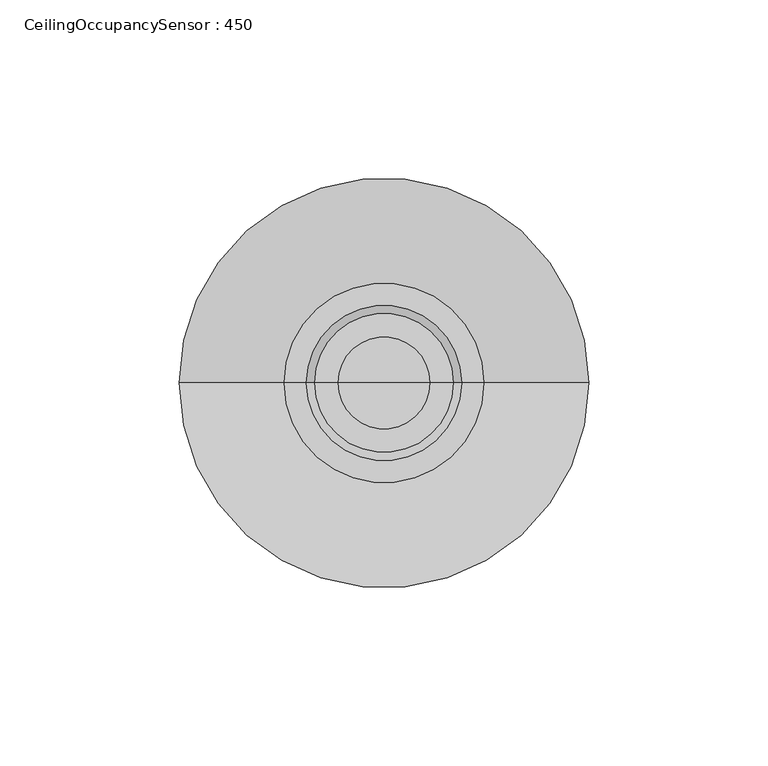
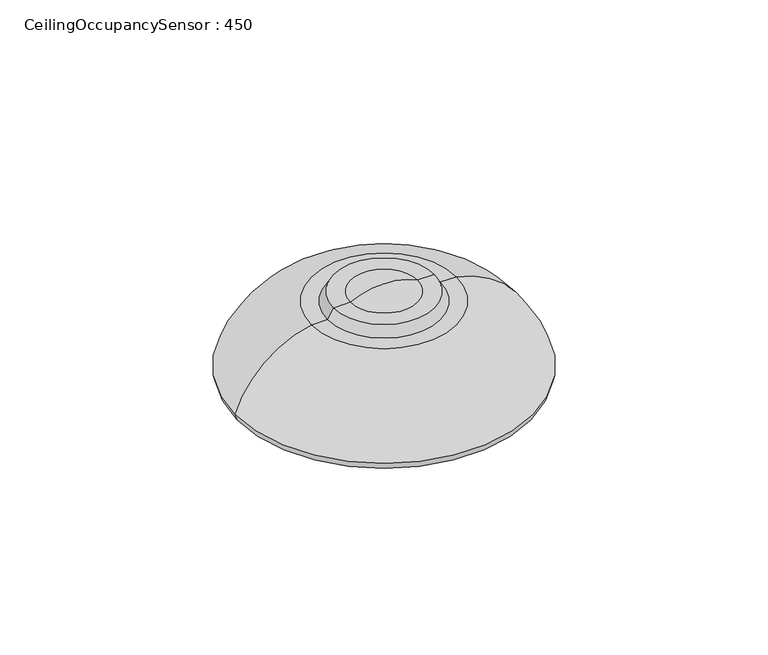
"""IFC4 building model written with IfcOpenShell, lengths in millimetres: switching device geometry, CeilingOccupancySensor : 450."""

from ifc_helpers import new_model, si_unit, point, frame, origin, origin_with_axes, place, context, project, spatial, polyline, circle_curve, ellipse_curve, trimmed, source, transform, mapped, element, save
from ifc_brep_helpers import plane_surface, revolved_surface, advanced_brep


def ceilingoccupancysensor_450_02cbfb90(model_context):
    return source(origin(), model_context, "Body", "AdvancedBrep", [
        advanced_brep(
        [(-12.7998992, 0.0, 32.54375), (12.7998992, 0.0, 32.54375), (0.0, 0.0, 35.5203125), (-19.3725919, 0.0, 32.54375), (19.3725919, 0.0, 32.54375), (-21.6519708, 0.0, 28.5957499), (21.6519708, 0.0, 28.5957499), (-27.834758, 0.0, 28.5957499), (27.834758, 0.0, 28.5957499), (-57.15, 0.0, 2.3911967), (57.15, 0.0, 2.3911967), (-56.5092808, 0.0, 0.0), (56.5092808, 0.0, 0.0), (0.0, 0.0, 0.0)],
        [
            (0, 1, circle_curve(frame((0.0, 0.0, 32.54375), z_axis=(0.0, 0.0, 1.0), x_axis=(1.0, 0.0, 0.0)), 12.7998992)),
            (1, 2, circle_curve(frame((0.750087, 0.0, 9.7363307), z_axis=(0.0, -1.0, 0.0), x_axis=(1.0, 0.0, 0.0)), 25.79489)),
            (2, 0, circle_curve(frame((-0.750087, 0.0, 9.7363307), z_axis=(0.0, -1.0, 0.0), x_axis=(-1.0, 0.0, 0.0)), 25.79489)),
            (1, 0, circle_curve(frame((0.0, 0.0, 32.54375), z_axis=(0.0, 0.0, 1.0), x_axis=(1.0, 0.0, 0.0)), 12.7998992)),
            (3, 4, circle_curve(frame((0.0, 0.0, 32.54375), z_axis=(0.0, 0.0, 1.0), x_axis=(1.0, 0.0, 0.0)), 19.3725919)),
            (4, 1),
            (0, 3),
            (4, 3, circle_curve(frame((0.0, 0.0, 32.54375), z_axis=(0.0, 0.0, 1.0), x_axis=(1.0, 0.0, 0.0)), 19.3725919)),
            (5, 6, circle_curve(frame((0.0, 0.0, 28.5957499), z_axis=(0.0, 0.0, 1.0), x_axis=(1.0, 0.0, 0.0)), 21.6519708)),
            (6, 4),
            (3, 5),
            (6, 5, circle_curve(frame((0.0, 0.0, 28.5957499), z_axis=(0.0, 0.0, 1.0), x_axis=(1.0, 0.0, 0.0)), 21.6519708)),
            (7, 8, circle_curve(frame((0.0, 0.0, 28.5957499), z_axis=(0.0, 0.0, 1.0), x_axis=(1.0, 0.0, 0.0)), 27.834758)),
            (8, 6),
            (5, 7),
            (8, 7, circle_curve(frame((0.0, 0.0, 28.5957499), z_axis=(0.0, 0.0, 1.0), x_axis=(1.0, 0.0, 0.0)), 27.834758)),
            (9, 10, circle_curve(frame((0.0, 0.0, 2.3911967), z_axis=(0.0, 0.0, 1.0), x_axis=(1.0, 0.0, 0.0)), 57.15)),
            (10, 8, circle_curve(frame((20.1846327, 0.0, -9.4623798), z_axis=(0.0, -1.0, 0.0), x_axis=(1.0, 0.0, 0.0)), 38.8193979)),
            (7, 9, circle_curve(frame((-20.1846327, 0.0, -9.4623798), z_axis=(0.0, -1.0, 0.0), x_axis=(-1.0, 0.0, 0.0)), 38.8193979)),
            (10, 9, circle_curve(frame((0.0, 0.0, 2.3911967), z_axis=(0.0, 0.0, 1.0), x_axis=(1.0, 0.0, 0.0)), 57.15)),
            (11, 12, circle_curve(origin_with_axes(), 56.5092808)),
            (12, 10),
            (9, 11),
            (12, 11, circle_curve(origin_with_axes(), 56.5092808)),
            (13, 12),
            (11, 13),
        ],
        [
            revolved_surface(trimmed(ellipse_curve(frame((0.750087, 0.0, 9.7363307), z_axis=(0.0, 1.0, 0.0), x_axis=(1.0, 0.0, 0.0)), 25.79489, 25.79489), [point((0.0, 0.0, 35.5203125))], [point((12.7998992, 0.0, 32.54375))], True, "CARTESIAN"), (0.0, 0.0, 38.1), (0.0, 0.0, -1.0)),
            plane_surface(frame((0.0, 0.0, 32.54375), z_axis=(0.0, 0.0, 1.0), x_axis=(1.0, 0.0, 0.0))),
            revolved_surface(polyline([(19.3725919, 0.0, 32.54375), (21.6519708, 0.0, 28.5957499)]), (0.0, 0.0, 38.1), (0.0, 0.0, -1.0)),
            plane_surface(frame((0.0, 0.0, 28.5957499), z_axis=(0.0, 0.0, 1.0), x_axis=(1.0, 0.0, 0.0))),
            revolved_surface(trimmed(ellipse_curve(frame((20.1846327, 0.0, -9.4623798), z_axis=(0.0, 1.0, 0.0), x_axis=(1.0, 0.0, 0.0)), 38.8193979, 38.8193979), [point((27.834758, 0.0, 28.5957499))], [point((57.15, 0.0, 2.3911967))], True, "CARTESIAN"), (0.0, 0.0, 38.1), (0.0, 0.0, -1.0)),
            revolved_surface(polyline([(57.15, 0.0, 2.3911967), (56.5092808, 0.0, 0.0)]), (0.0, 0.0, 38.1), (0.0, 0.0, -1.0)),
            plane_surface(frame((0.0, 0.0, 0.0), z_axis=(0.0, 0.0, -1.0), x_axis=(1.0, 0.0, 0.0))),
        ],
        [
            (0, [[1, 2, 3]]),
            (0, [[4, -3, -2]]),
            (1, [[5, 6, -1, 7]]),
            (1, [[8, -7, -4, -6]]),
            (2, [[9, 10, -5, 11]]),
            (2, [[12, -11, -8, -10]]),
            (3, [[13, 14, -9, 15]]),
            (3, [[16, -15, -12, -14]]),
            (4, [[17, 18, -13, 19]]),
            (4, [[20, -19, -16, -18]]),
            (5, [[21, 22, -17, 23]]),
            (5, [[24, -23, -20, -22]]),
            (6, [[25, -21, 26]]),
            (6, [[-26, -24, -25]]),
        ],
    ),
    ])


if __name__ == "__main__":
    model = new_model("IFC4")
    model_context = context("Model", 3, world=origin())
    ifc_project = project(units=[si_unit("LENGTHUNIT", "METRE", prefix="MILLI")], contexts=[model_context])
    site = spatial("IfcSite", under=ifc_project)
    building = spatial("IfcBuilding", under=site)
    placement = place(None, origin())
    ceilingoccupancysensor_450_shape = ceilingoccupancysensor_450_02cbfb90(model_context)
    element("IfcSwitchingDevice", 1, ObjectType="CeilingOccupancySensor : 450", at=placement, inside=building, context=model_context, shape_type="MappedRepresentation", body=[
        mapped(ceilingoccupancysensor_450_shape, transform((0.0, 0.0, 0.0), x_axis=(1.0, 0.0, 0.0), y_axis=(0.0, 1.0, 0.0), z_axis=(0.0, 0.0, 1.0))),
    ])
    save(model, "model.ifc")

# Revit data of these elements
# Project information
#   Author = "F.W."
#   Classification.Facility.Description = "Mixed-Gender Dormitory"
#   Classification.Facility.Number = "11-16 27 14"
#   COBie.CreatedBy = "info@mma.ie"
#   COBie.CreatedOn = "2017-07-25T10:15:16"
#   COBie.Facility.Name = "EDTP-001"
#   COBie.Facility.Category = "11-16 27 14 : Mixed-Gender Dormitory"
#   COBie.Facility.ProjectName = "East Dormitory Project"
#   COBie.Facility.SiteName = "East Healey Street, Champaign, Illiniois USA"
#   COBie.Facility.LinearUnits = "Millimeters"
#   COBie.Facility.AreaUnits = "Square Meters"
#   COBie.Facility.VolumeUnits = "Cubic Meters"
#   COBie.Facility.CurrencyUnit = "Dollar"
#   COBie.Facility.AreaMeasurement = "Revit Default Area Calculation Method"
#   COBie.Facility.Description = "Two Story, Luxury Dormitory"
#   COBie.Facility.ProjectDescription = "One of Four Dormitories on the E.Healey Site"
#   COBie.Facility.SiteDescription = "Four Dormitories Project Site"
#   COBie.Facility.Phase = "60% Design Submission"
#   Project Issue Date = "Issue Date"
#   Project Status = "Final Issue"
#   Client Name = "Prairie Sky Consulting"
#   Project Address = "East Healey Street,\nChampaign,\nIllinois,\nUSA."
#   Project Name = "Four Dormitory Complex"
#   Project Number = "East Dormitory"
# Type "CeilingOccupancySensor : 450"
#   Type Mark = "CeilingOccupancySensor"
#   Classification.OmniClass.21.Number = "21-04 50 40 10"
#   Classification.OmniClass.21.Description = "Lighting Control"
#   Classification.UniFormat.II.Description = "Lighting Control"
#   Classification.OmniClass.23.Number = "23-29 11 23 17"
#   Classification.OmniClass.23.Description = "Intrusion Detection Photoelectric Sensors"
#   Classification.UniFormat.II.Number = "D5040.10"
#   COBie.Type.CreatedBy = "info@mma.ie"
#   COBie.Type.CreatedOn = "2017-07-25T10:15:16"
#   COBie.Type.Name = "CeilingOccupancySensor"
#   COBie.Type.Category = "23-29 11 23 17 : Intrusion Detection Photoelectric Sensors"
#   COBie.Type.Description = "CeilingOccupancySensor_450"
#   COBie.Type.AssetType = "Fixed"
#   COBie.Type.Manufacturer = ""
#   COBie.Type.ModelNumber = ""
#   Voltage Comments = "20-24VDC"
#   Series = ""
#   Product URL = ""
#   Keynote = "28 16 19.A"
#   Copyright = ""
#   CADworks URL = ""
#   C.O.S. Material = "Plastic-White-Gloss"
#   Assembly Code = "D5030800"
#   COBie.Type.ReplacementCost = 0
#   Switch Voltage = 230 V
#   Nominal Width = 114.3 mm
#   Nominal Length = 114.3 mm
#   Nominal Depth = 35.52 mm
#   Minor Motion Detection = 1981.2 mm
#   Major Motion Detection = 3657.6 mm
#   Field of View = 360.00°
#   Coverage = 41.8064 m²
#   C.O.S. Field of View = 360.00°
#   C.O.S. Coverage = 41.8064 m²
#   COBie.Type = yes
#   Light Source [instance default] = yes
#   Infrared Minor Motion [instance default] = no
#   Infrared Major Motion [instance default] = no
#   Ballast Number of Poles = 1
#   Sensor Material = Plastic-White-Gloss
#   URL = ""
#   Type Comments = ""
#   Model = ""
#   Manufacturer = ""
#   Description = (empty or 0)
#   Default Elevation = 0
# Element 1 (IfcSwitchingDevice, "CeilingOccupancySensor : 450")
#   Materials on its faces: "Plastic-White-Gloss"
# Materials
#   "Plastic-White-Gloss": class "Plastic", colour RGB 255 255 255, transparency 0, Cost = 0
